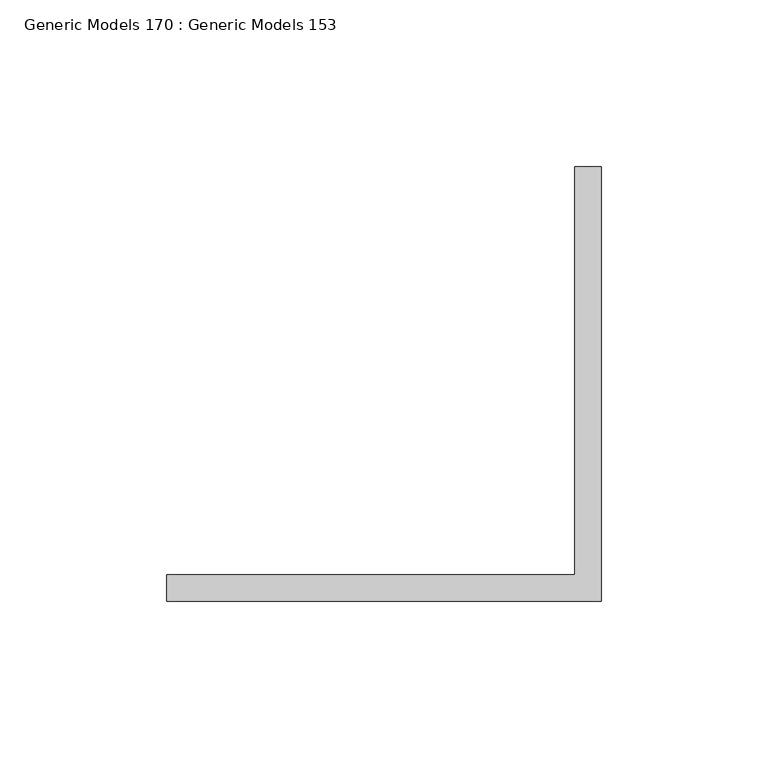
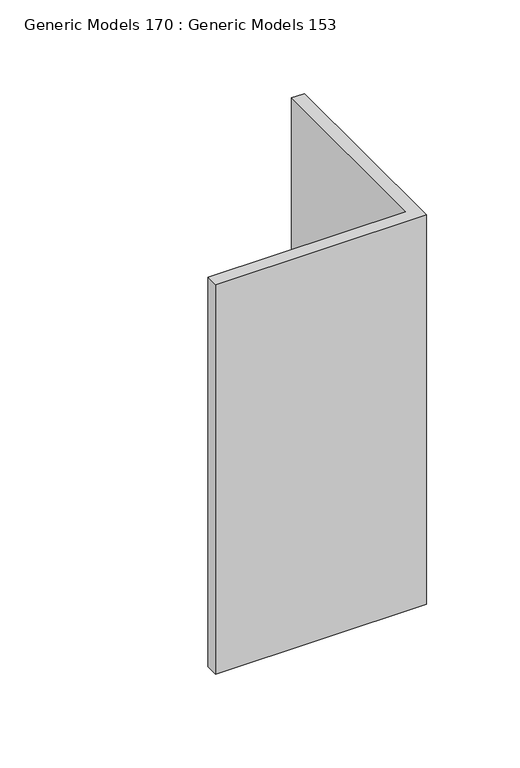
"""IFC4 building model written with IfcOpenShell, lengths in millimetres: proxy geometry, Generic Models 170 : Generic Models 153."""

from ifc_helpers import new_model, si_unit, frame, origin, place, context, project, spatial, polyline, outline, extrude, source, transform, mapped, element, save


def generic_models_170_generic_models_153_db2765b9(model_context):
    return source(origin(), model_context, "Body", "SweptSolid", [
        extrude(outline(polyline([(31762.6846032, 30974.3656612), (31770.6221032, 30974.3656612), (31770.6221032, 30844.1906612), (31640.4471032, 30844.1906612), (31640.4471032, 30852.1281612), (31762.6846032, 30852.1281612), (31762.6846032, 30974.3656612)])), frame((0.0, 0.0, 271626.0125), z_axis=(0.0, 0.0, 1.0), x_axis=(1.0, 0.0, 0.0)), (0.0, 0.0, 1.0), 254.0),
    ])


if __name__ == "__main__":
    model = new_model("IFC4")
    model_context = context("Model", 3, world=origin())
    ifc_project = project(units=[si_unit("LENGTHUNIT", "METRE", prefix="MILLI")], contexts=[model_context])
    site = spatial("IfcSite", under=ifc_project)
    building = spatial("IfcBuilding", under=site)
    placement = place(None, origin())
    generic_models_170_generic_models_153_shape = generic_models_170_generic_models_153_db2765b9(model_context)
    element("IfcBuildingElementProxy", 1, Name="Generic Models 170 : Generic Models 153", ObjectType="Generic Models 170 : Generic Models 153", at=placement, inside=building, context=model_context, shape_type="MappedRepresentation", body=[
        mapped(generic_models_170_generic_models_153_shape, transform((0.0, 0.0, 0.0), x_axis=(1.0, 0.0, 0.0), y_axis=(0.0, 1.0, 0.0), z_axis=(0.0, 0.0, 1.0))),
    ])
    save(model, "model.ifc")
